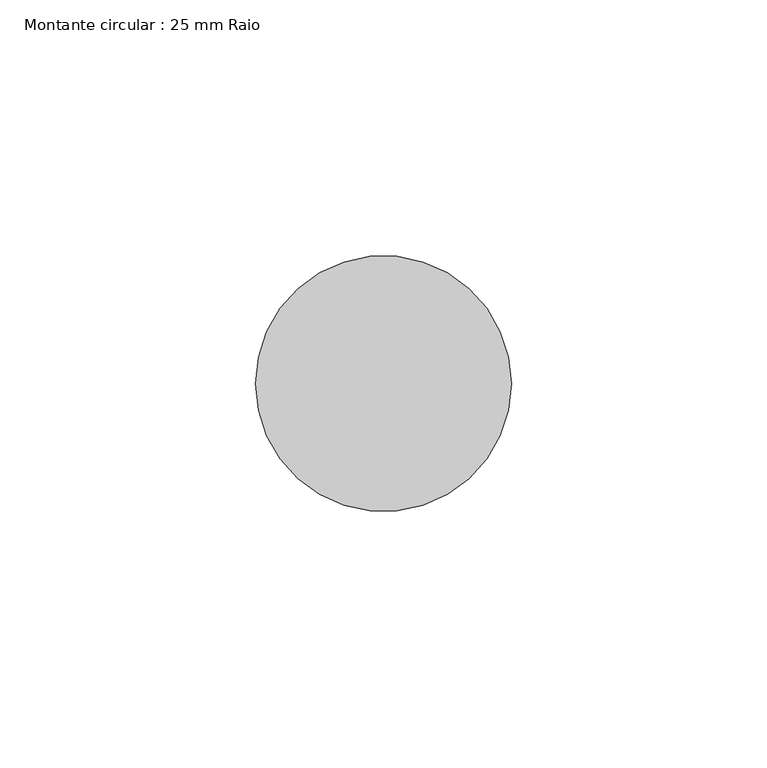
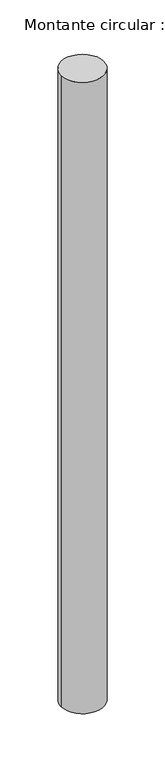
"""IFC4 building model written with IfcOpenShell, lengths in millimetres: member geometry, Montante circular : 25 mm Raio."""

from ifc_helpers import new_model, si_unit, point, frame, origin, origin_2d, place, context, project, spatial, circle_curve, trimmed, segment, composite_curve, outline, extrude, source, transform, mapped, element, save


def montante_circular_25_mm_raio_0640af2a(model_context):
    return source(origin(), model_context, "Body", "SweptSolid", [
        extrude(outline(composite_curve([segment(trimmed(circle_curve(origin_2d(), 25.0), [point((25.0, 0.0))], [point((-25.0, 0.0))], False, "CARTESIAN"), True, "CONTINUOUS"), segment(trimmed(circle_curve(origin_2d(), 25.0), [point((-25.0, 0.0))], [point((25.0, 0.0))], False, "CARTESIAN"), True, "CONTINUOUS")], self_intersect=False)), frame((0.0, 0.0, -784.0519788), z_axis=(0.0, 0.0, 1.0), x_axis=(1.0, 0.0, 0.0)), (0.0, 0.0, 1.0), 784.0519788),
    ])


if __name__ == "__main__":
    model = new_model("IFC4")
    model_context = context("Model", 3, world=origin())
    ifc_project = project(units=[si_unit("LENGTHUNIT", "METRE", prefix="MILLI")], contexts=[model_context])
    site = spatial("IfcSite", under=ifc_project)
    building = spatial("IfcBuilding", under=site)
    placement = place(None, origin())
    montante_circular_25_mm_raio_shape = montante_circular_25_mm_raio_0640af2a(model_context)
    element("IfcMember", 1, ObjectType="Montante circular : 25 mm Raio", at=placement, inside=building, context=model_context, shape_type="MappedRepresentation", body=[
        mapped(montante_circular_25_mm_raio_shape, transform((0.0, 0.0, 0.0), x_axis=(1.0, 0.0, 0.0), y_axis=(0.0, 1.0, 0.0), z_axis=(0.0, 0.0, 1.0))),
    ])
    save(model, "model.ifc")

# Revit data of these elements
# Type "Montante circular : 25 mm Raio"
#   built-in parameter 1007350 = 0.082021 (stored number, unit not read)
# Element 1 (IfcMember, "Montante circular : 25 mm Raio")
#   Materials on its faces: "Alumín."
# Materials
#   "Alumín.": class "Metal", colour RGB 247 247 247, transparency 0, Description = "Alumín. 6061", Cost = 0
